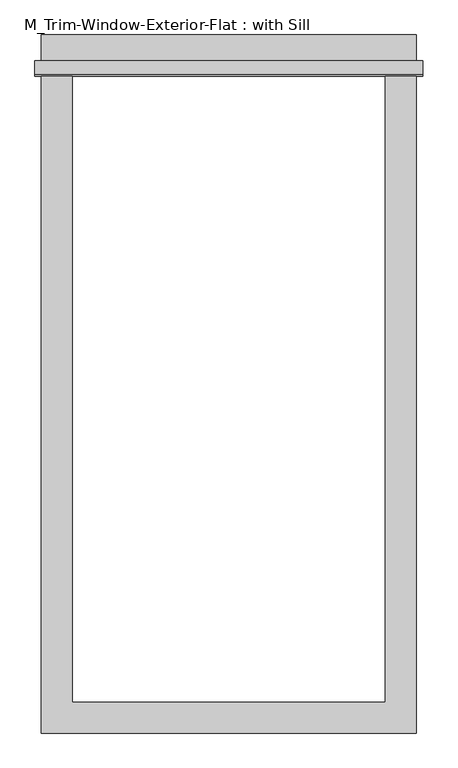
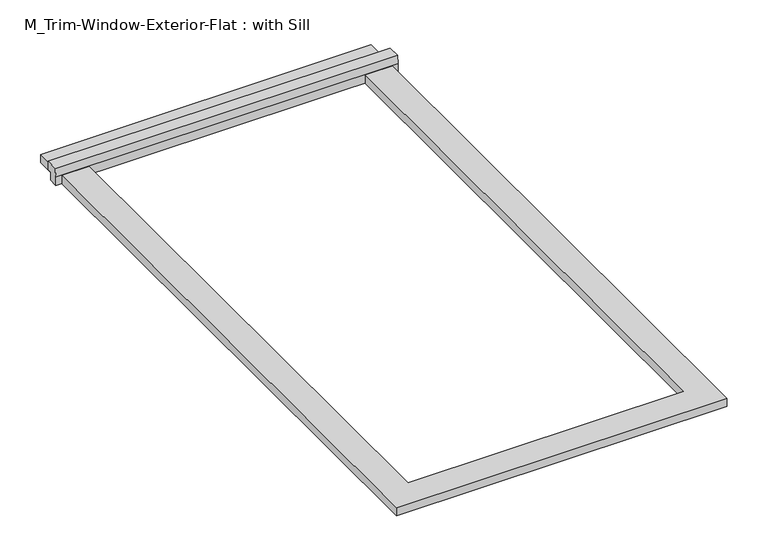
"""IFC4 building model written with IfcOpenShell, lengths in millimetres: proxy geometry, M_Trim-Window-Exterior-Flat : with Sill."""

from ifc_helpers import new_model, si_unit, frame, origin, origin_with_axes, place, context, project, spatial, polyline, outline, extrude, source, transform, mapped, element, save


def m_trim_window_exterior_flat_with_sill_620770e2(model_context):
    return source(origin(), model_context, "Body", "SweptSolid", [
        extrude(outline(polyline([(364.8, 1239.6323709), (-364.8, 1239.6323709), (-364.8, 1299.6323709), (364.8, 1299.6323709), (364.8, 1239.6323709)])), origin_with_axes(), (0.0, 0.0, 1.0), 19.05),
        extrude(outline(polyline([(1249.2, 38.1), (1249.2, 19.05), (1239.6323709, 19.05), (1239.6323709, 0.0), (1219.2, 0.0), (1219.2, 19.05), (1221.6580645, 38.1), (1249.2, 38.1)])), frame((-377.5, 0.0, 0.0), z_axis=(1.0, 0.0, 0.0), x_axis=(0.0, 1.0, 0.0)), (0.0, 0.0, 1.0), 755.0),
        extrude(outline(polyline([(-364.8, -60.0), (-364.8, 1219.2), (-304.8, 1219.2), (-304.8, 0.0), (304.8, 0.0), (304.8, 1219.2), (364.8, 1219.2), (364.8, -60.0), (-364.8, -60.0)])), origin_with_axes(), (0.0, 0.0, 1.0), 19.05),
    ])


if __name__ == "__main__":
    model = new_model("IFC4")
    model_context = context("Model", 3, world=origin())
    ifc_project = project(units=[si_unit("LENGTHUNIT", "METRE", prefix="MILLI")], contexts=[model_context])
    site = spatial("IfcSite", under=ifc_project)
    building = spatial("IfcBuilding", under=site)
    placement = place(None, origin())
    m_trim_window_exterior_flat_with_sill_shape = m_trim_window_exterior_flat_with_sill_620770e2(model_context)
    element("IfcBuildingElementProxy", 1, Name="M_Trim-Window-Exterior-Flat : with Sill", ObjectType="M_Trim-Window-Exterior-Flat : with Sill", at=placement, inside=building, context=model_context, shape_type="MappedRepresentation", body=[
        mapped(m_trim_window_exterior_flat_with_sill_shape, transform((0.0, 0.0, 0.0), x_axis=(1.0, 0.0, 0.0), y_axis=(0.0, 1.0, 0.0), z_axis=(0.0, 0.0, 1.0))),
    ])
    save(model, "model.ifc")

# Revit data of these elements
# Type "M_Trim-Window-Exterior-Flat : with Sill"
#   Trim Width = 0' - 2.3622"
#   Trim Thickness_Picture Frame = 0' - 1.1811"
#   Trim Thickness_with Sill = 0' - 0 3/4"
#   Sill Thickness = 0' - 1.1811"
#   Opening Width [instance default] = 1' - 11.62205"
#   Opening Height [instance default] = 2' - 11.43307"
#   Default Elevation = 3' - 11.24409"
#   Sill = yes
#   Picture Frame = no
#   Trim Material [instance default] = none
# Element 1 (IfcBuildingElementProxy, "M_Trim-Window-Exterior-Flat : with Sill")
#   Opening Width = 2' - 0"
#   Opening Height = 4' - 0"
#   Trim Material = Clad - White
#   Materials on its faces: "Clad - White"
# Materials
#   "Clad - White": class "Wood", colour RGB 242 242 238, transparency 0, Cost = 0
